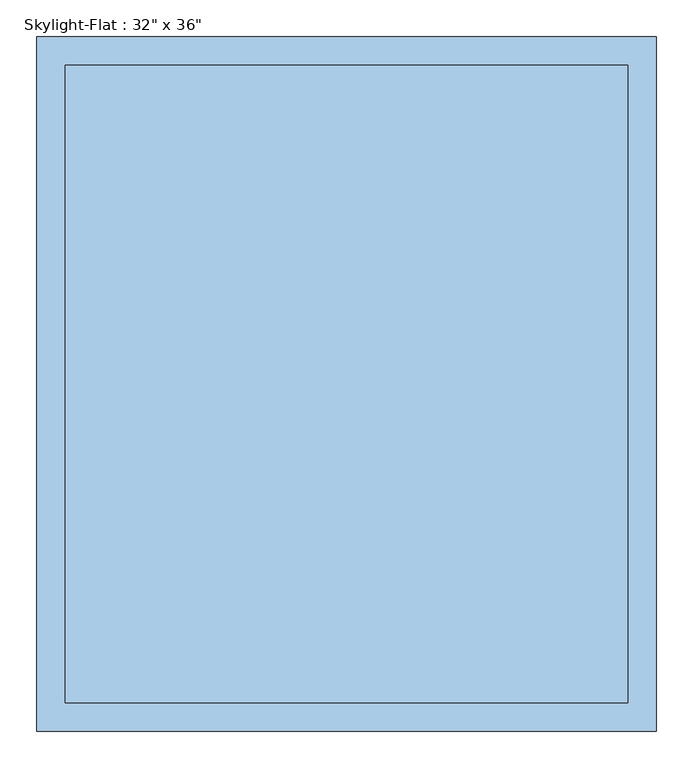
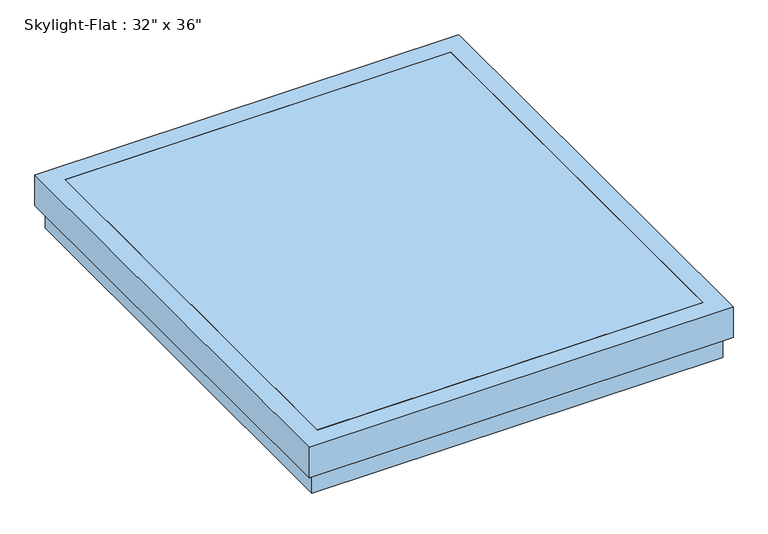
"""IFC4 building model written with IfcOpenShell, lengths in millimetres: window geometry."""

import ifcopenshell
import ifcopenshell.guid

model = None  # the IFC model being written
_history = None  # IfcOwnerHistory: only IFC2X3 demands one
_inside = {}  # id of a spatial element -> (the spatial element, [elements in it])
_under = {}  # id of a project, library or spatial element -> (it, [spatial elements below it])
_declared = {}  # id of a project -> (the project, [libraries it declares])
_typed = {}  # id of a type object -> (the type object, [elements of that type])
_made_of = {}  # id of a material, layer set ... -> (it, [elements and type objects made of it])


def new_model(schema):
    """Start an empty IFC model of exactly this schema.

    Asked for "IFC4X3", IfcOpenShell would pick the latest addendum, in which some entities
    have other attributes; the version numbers below select the first issue.
    IFC2X3 requires an IfcOwnerHistory on every rooted entity: one is made here for all.
    """
    global model, _history
    if schema == "IFC4X3":
        model = ifcopenshell.file(schema_version=(4, 3, 0, 0))
    else:
        model = ifcopenshell.file(schema=schema)
    _inside.clear()
    _under.clear()
    _declared.clear()
    _typed.clear()
    _made_of.clear()
    _history = None
    if model.schema == "IFC2X3":
        org = make("IfcOrganization", Name="unknown")
        user = make(
            "IfcPersonAndOrganization",
            ThePerson=make("IfcPerson", FamilyName="unknown"),
            TheOrganization=org,
        )
        app = make(
            "IfcApplication",
            ApplicationDeveloper=org,
            Version="unknown",
            ApplicationFullName="unknown",
            ApplicationIdentifier="unknown",
        )
        _history = make(
            "IfcOwnerHistory",
            OwningUser=user,
            OwningApplication=app,
            ChangeAction="ADDED",
            CreationDate=0,
        )
    return model


def make(cls, **values):
    """One entity of the class cls with the attributes given. An attribute that is None is left unset."""
    return model.create_entity(
        cls, **{name: value for name, value in values.items() if value is not None}
    )


def rooted(cls, **values):
    """An entity with a GlobalId (a new one), such as an element, a storey or a relation."""
    return make(cls, GlobalId=ifcopenshell.guid.new(), OwnerHistory=_history, **values)


def si_unit(unit_type, name, prefix=None):
    """IfcSIUnit, for example si_unit("LENGTHUNIT", "METRE", prefix="MILLI")."""
    return make("IfcSIUnit", UnitType=unit_type, Prefix=prefix, Name=name)


def assignment(units):
    """IfcUnitAssignment: the units of a project."""
    return None if units is None else make("IfcUnitAssignment", Units=units)


def point(xyz):
    """IfcCartesianPoint."""
    return None if xyz is None else make("IfcCartesianPoint", Coordinates=xyz)


def direction(xyz):
    """IfcDirection."""
    return None if xyz is None else make("IfcDirection", DirectionRatios=xyz)


def frame(location, z_axis=None, x_axis=None):
    """IfcAxis2Placement3D, a coordinate frame: its origin and axes. An axis left out is left unset."""
    return make(
        "IfcAxis2Placement3D",
        Location=point(location),
        Axis=direction(z_axis),
        RefDirection=direction(x_axis),
    )


def origin():
    """The frame at (0, 0, 0) with its axes left unset."""
    return frame((0.0, 0.0, 0.0))


def place(relative_to, where):
    """IfcLocalPlacement: puts the frame where relative to a parent placement (None: the world)."""
    return make(
        "IfcLocalPlacement", PlacementRelTo=relative_to, RelativePlacement=where
    )


def context(
    kind, dimensions, precision=None, world=None, true_north=None, identifier=None
):
    """IfcGeometricRepresentationContext, for example the 3D "Model" context."""
    return make(
        "IfcGeometricRepresentationContext",
        ContextIdentifier=identifier,
        ContextType=kind,
        CoordinateSpaceDimension=dimensions,
        Precision=precision,
        WorldCoordinateSystem=world,
        TrueNorth=true_north,
    )


def project(units=None, contexts=None):
    """IfcProject with its units and contexts."""
    return rooted(
        "IfcProject",
        Name="project",
        RepresentationContexts=contexts,
        UnitsInContext=assignment(units),
    )


def spatial(cls, under=None, at=None, **own):
    """A site, building, storey or space (cls), placed at a placement, below another one or the project."""
    s = rooted(cls, ObjectPlacement=at, **own)
    if under is not None:
        _under.setdefault(under.id(), (under, []))[1].append(s)
    return s


def polyline(points):
    """IfcPolyline through the points."""
    return make("IfcPolyline", Points=[point(p) for p in points])


def outline(outer, holes=None, kind="AREA"):
    """IfcArbitraryClosedProfileDef: a profile drawn as a closed curve; with holes, ...WithVoids."""
    if holes is None:
        return make("IfcArbitraryClosedProfileDef", ProfileType=kind, OuterCurve=outer)
    return make(
        "IfcArbitraryProfileDefWithVoids",
        ProfileType=kind,
        OuterCurve=outer,
        InnerCurves=holes,
    )


def extrude(swept, where, along, depth):
    """IfcExtrudedAreaSolid: the profile swept, set in the frame where, extruded along a direction by depth."""
    return make(
        "IfcExtrudedAreaSolid",
        SweptArea=swept,
        Position=where,
        ExtrudedDirection=direction(along),
        Depth=depth,
    )


def faces_of(points, faces, orient=None, outer=None):
    """IfcFace entities. A face is a list of loops; a loop is a list of indices into points, from 0.

    orient and outer hold one flag for each loop. By default every Orientation is true, the
    first loop of a face is its IfcFaceOuterBound and the others are IfcFaceBound.
    """
    made = []
    for i, loops in enumerate(faces):
        bounds = []
        for j, loop in enumerate(loops):
            is_outer = j == 0 if outer is None else outer[i][j]
            bounds.append(
                make(
                    "IfcFaceOuterBound" if is_outer else "IfcFaceBound",
                    Bound=make("IfcPolyLoop", Polygon=[points[k] for k in loop]),
                    Orientation=True if orient is None else orient[i][j],
                )
            )
        made.append(make("IfcFace", Bounds=bounds))
    return made


def faceted_brep(points, faces, orient=None, outer=None, voids=None):
    """IfcFacetedBrep: a solid bounded by flat faces; with voids (closed shells), ...WithVoids."""
    shared = [point(p) for p in points]
    hull = make("IfcClosedShell", CfsFaces=faces_of(shared, faces, orient, outer))
    if voids is None:
        return make("IfcFacetedBrep", Outer=hull)
    return make(
        "IfcFacetedBrepWithVoids",
        Outer=hull,
        Voids=[
            make(cls, CfsFaces=faces_of(shared, fs, o, b)) for cls, fs, o, b in voids
        ],
    )


def shape(context_of_items, identifier, shape_type, items):
    """IfcShapeRepresentation: the items that make up one representation, for example the "Body"."""
    return make(
        "IfcShapeRepresentation",
        ContextOfItems=context_of_items,
        RepresentationIdentifier=identifier,
        RepresentationType=shape_type,
        Items=items,
    )


def source(mapping_origin, context_of_items, identifier, shape_type, items):
    """IfcRepresentationMap: a shape defined once, which mapped items show again and again."""
    return make(
        "IfcRepresentationMap",
        MappingOrigin=mapping_origin,
        MappedRepresentation=shape(context_of_items, identifier, shape_type, items),
    )


def transform(
    local_origin,
    x_axis=None,
    y_axis=None,
    z_axis=None,
    scale=None,
    scale2=None,
    scale3=None,
    uniform=True,
):
    """IfcCartesianTransformationOperator3D, or its non-uniform kind. x_axis, y_axis, z_axis: its Axis1, 2, 3."""
    if uniform:
        return make(
            "IfcCartesianTransformationOperator3D",
            Axis1=direction(x_axis),
            Axis2=direction(y_axis),
            LocalOrigin=point(local_origin),
            Scale=scale,
            Axis3=direction(z_axis),
        )
    return make(
        "IfcCartesianTransformationOperator3DnonUniform",
        Axis1=direction(x_axis),
        Axis2=direction(y_axis),
        LocalOrigin=point(local_origin),
        Scale=scale,
        Axis3=direction(z_axis),
        Scale2=scale2,
        Scale3=scale3,
    )


def mapped(mapping_source, mapping_target):
    """IfcMappedItem: shows the shape of a source again, moved by a transform."""
    return make(
        "IfcMappedItem", MappingSource=mapping_source, MappingTarget=mapping_target
    )


def made_of(thing, what):
    """Note that an element or type object is made of a material, layer set ...; save() writes the relation."""
    if what is not None:
        _made_of.setdefault(what.id(), (what, []))[1].append(thing)
    return thing


def element(
    cls,
    number,
    at=None,
    inside=None,
    cuts=None,
    type_object=None,
    material=None,
    context=None,
    identifier="Body",
    shape_type=None,
    held_by="IfcProductDefinitionShape",
    body=None,
    shapes=None,
    **own,
):
    """One element of the class cls, such as IfcWall. Its Tag is "e" and its number.

    at: its placement. inside: the storey or other place that contains it. cuts: it is an
    opening in that element (IfcRelVoidsElement). A single representation is given by context,
    identifier, shape_type and body (its items); several are given by shapes. held_by: the class
    of the entity that holds the representations. save() writes the other relations.
    """
    e = rooted(cls, Tag="e%d" % number, ObjectPlacement=at, **own)
    if body is not None:
        shapes = [shape(context, identifier, shape_type, body)]
    if shapes is not None:
        e.Representation = make(held_by, Representations=shapes)
    if inside is not None:
        _inside.setdefault(inside.id(), (inside, []))[1].append(e)
    if cuts is not None:
        rooted(
            "IfcRelVoidsElement", RelatingBuildingElement=cuts, RelatedOpeningElement=e
        )
    if type_object is not None:
        _typed.setdefault(type_object.id(), (type_object, []))[1].append(e)
    return made_of(e, material)


def aggregate(whole, parts):
    """IfcRelAggregates: a whole, such as a stair, and the parts it consists of."""
    return rooted("IfcRelAggregates", RelatingObject=whole, RelatedObjects=parts)


def save(model, path):
    """Write the relations noted so far, then the file.

    IfcRelAggregates (storeys below a building ...), IfcRelContainedInSpatialStructure (elements
    in a storey), IfcRelDefinesByType, IfcRelAssociatesMaterial and IfcRelDeclares: one each for
    every whole, place, type object, material and project.
    """
    for whole, parts in _under.values():
        aggregate(whole, parts)
    for where, things in _inside.values():
        rooted(
            "IfcRelContainedInSpatialStructure",
            RelatedElements=things,
            RelatingStructure=where,
        )
    for kind, things in _typed.values():
        rooted("IfcRelDefinesByType", RelatedObjects=things, RelatingType=kind)
    for what, things in _made_of.values():
        rooted("IfcRelAssociatesMaterial", RelatedObjects=things, RelatingMaterial=what)
    for by, libraries in _declared.values():
        rooted("IfcRelDeclares", RelatingContext=by, RelatedDefinitions=libraries)
    model.write(path)


def window_a8ca25b6(model_context):
    return source(origin(), model_context, "Body", "SolidModel", [
        extrude(outline(polyline([(381.0, 431.8), (381.0, -431.8), (-381.0, -431.8), (-381.0, 431.8), (381.0, 431.8)])), frame((0.0, 0.0, 3966.36875), z_axis=(0.0, 0.0, 1.0), x_axis=(1.0, 0.0, 0.0)), (0.0, 0.0, 1.0), 5.55625),
        faceted_brep([(419.1, 469.9, 3908.425), (419.1, 469.9, 3971.925), (419.1, -469.9, 3971.925), (419.1, -469.9, 3908.425), (406.4, 457.2, 3946.525), (406.4, 457.2, 3908.425), (406.4, -457.2, 3908.425), (406.4, -457.2, 3946.525), (381.0, 431.8, 3971.925), (381.0, 431.8, 3946.525), (381.0, -431.8, 3946.525), (381.0, -431.8, 3971.925), (-419.1, -469.9, 3971.925), (-419.1, -469.9, 3908.425), (-406.4, -457.2, 3908.425), (-406.4, -457.2, 3946.525), (-381.0, -431.8, 3946.525), (-381.0, -431.8, 3971.925), (-419.1, 469.9, 3971.925), (-419.1, 469.9, 3908.425), (-406.4, 457.2, 3908.425), (-406.4, 457.2, 3946.525), (-381.0, 431.8, 3946.525), (-381.0, 431.8, 3971.925)], [[[0, 1, 2, 3]], [[4, 5, 6, 7]], [[8, 9, 10, 11]], [[3, 2, 12, 13]], [[7, 6, 14, 15]], [[11, 10, 16, 17]], [[13, 12, 18, 19]], [[15, 14, 20, 21]], [[17, 16, 22, 23]], [[1, 18, 12, 2], [11, 17, 23, 8]], [[19, 18, 1, 0]], [[3, 13, 19, 0], [5, 20, 14, 6]], [[21, 20, 5, 4]], [[7, 15, 21, 4], [9, 22, 16, 10]], [[23, 22, 9, 8]]]),
        faceted_brep([(406.4, 457.2, 3863.975), (406.4, 457.2, 3946.525), (406.4, -457.2, 3946.525), (406.4, -457.2, 3863.975), (342.9, 393.7, 3921.125), (342.9, 393.7, 3863.975), (342.9, -393.7, 3863.975), (342.9, -393.7, 3921.125), (381.0, 431.8, 3946.525), (381.0, 431.8, 3921.125), (381.0, -431.8, 3921.125), (381.0, -431.8, 3946.525), (-406.4, -457.2, 3946.525), (-406.4, -457.2, 3863.975), (-342.9, -393.7, 3863.975), (-342.9, -393.7, 3921.125), (-381.0, -431.8, 3921.125), (-381.0, -431.8, 3946.525), (-406.4, 457.2, 3946.525), (-406.4, 457.2, 3863.975), (-342.9, 393.7, 3863.975), (-342.9, 393.7, 3921.125), (-381.0, 431.8, 3921.125), (-381.0, 431.8, 3946.525)], [[[0, 1, 2, 3]], [[4, 5, 6, 7]], [[8, 9, 10, 11]], [[3, 2, 12, 13]], [[7, 6, 14, 15]], [[11, 10, 16, 17]], [[13, 12, 18, 19]], [[15, 14, 20, 21]], [[17, 16, 22, 23]], [[19, 18, 1, 0]], [[3, 13, 19, 0], [5, 20, 14, 6]], [[21, 20, 5, 4]], [[9, 22, 16, 10], [7, 15, 21, 4]], [[23, 22, 9, 8]], [[1, 18, 12, 2], [11, 17, 23, 8]]]),
    ])


if __name__ == "__main__":
    model = new_model("IFC4")
    model_context = context("Model", 3, world=origin())
    ifc_project = project(units=[si_unit("LENGTHUNIT", "METRE", prefix="MILLI")], contexts=[model_context])
    site = spatial("IfcSite", under=ifc_project)
    building = spatial("IfcBuilding", under=site)
    placement = place(None, origin())
    window_shape = window_a8ca25b6(model_context)
    element("IfcWindow", 1, ObjectType="Skylight-Flat : 32\" x 36\"", at=placement, inside=building, context=model_context, shape_type="MappedRepresentation", body=[
        mapped(window_shape, transform((0.0, 0.0, 0.0), x_axis=(1.0, 0.0, 0.0), y_axis=(0.0, 1.0, 0.0), z_axis=(0.0, 0.0, 1.0))),
    ])
    save(model, "model.ifc")

# Revit data of these elements
# Type "Skylight-Flat : 32\" x 36\""
#   Type Mark = "25"
#   Fire Rating = "0.5h"
#   Assembly Code = "B2020100"
#   Analytic Construction = "Single-glazed windows - domestic"
#   Width = 2' - 8"
#   Visual Light Transmittance = 0.9
#   Thermal Resistance (R) = 0.9899 (h·ft²·°F)/BTU
#   Solar Heat Gain Coefficient = 0.86
#   Rough Width = 2' - 8 1/2"
#   Rough Height = 3' - 0 1/2"
#   Height = 3' - 0"
#   Heat Transfer Coefficient (U) = 1.0102 BTU/(h·ft²·°F)
#   Base Height = 0' - 3 1/4"
#   Glass Panel Material = Glass
#   Frame Material = Metal - Bronze, Light Brush
# Element 1 (IfcWindow, "Skylight-Flat : 32\" x 36\"")
#   Materials on its faces: "Metal - Bronze, Light Brush", "Glass"
# Materials
#   "Glass": class "Glass", colour RGB 0 128 192, transparency 0.75, Description = "Soda Lime Glass", Cost = 0
#   "Metal - Bronze, Light Brush": class "Metal", colour RGB 113 80 70, transparency 0
